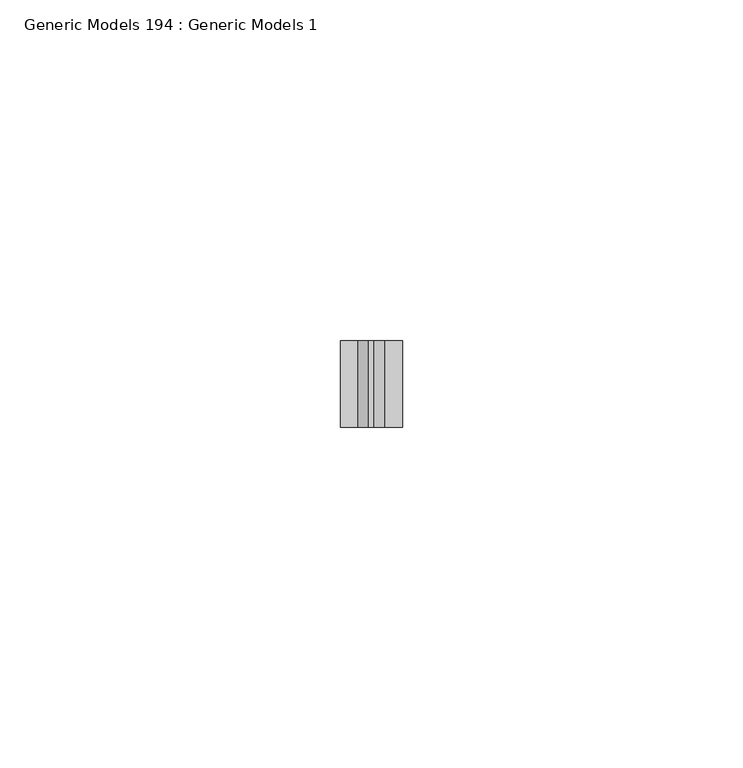
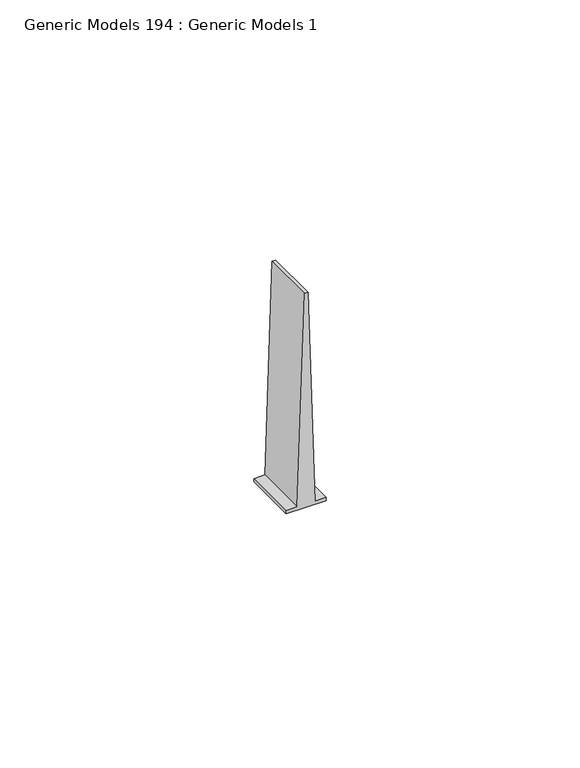
"""IFC4 building model written with IfcOpenShell, lengths in millimetres: proxy geometry, Generic Models 194 : Generic Models 1."""

import ifcopenshell
import ifcopenshell.guid

model = None  # the IFC model being written
_history = None  # IfcOwnerHistory: only IFC2X3 demands one
_inside = {}  # id of a spatial element -> (the spatial element, [elements in it])
_under = {}  # id of a project, library or spatial element -> (it, [spatial elements below it])
_declared = {}  # id of a project -> (the project, [libraries it declares])
_typed = {}  # id of a type object -> (the type object, [elements of that type])
_made_of = {}  # id of a material, layer set ... -> (it, [elements and type objects made of it])


def new_model(schema):
    """Start an empty IFC model of exactly this schema.

    Asked for "IFC4X3", IfcOpenShell would pick the latest addendum, in which some entities
    have other attributes; the version numbers below select the first issue.
    IFC2X3 requires an IfcOwnerHistory on every rooted entity: one is made here for all.
    """
    global model, _history
    if schema == "IFC4X3":
        model = ifcopenshell.file(schema_version=(4, 3, 0, 0))
    else:
        model = ifcopenshell.file(schema=schema)
    _inside.clear()
    _under.clear()
    _declared.clear()
    _typed.clear()
    _made_of.clear()
    _history = None
    if model.schema == "IFC2X3":
        org = make("IfcOrganization", Name="unknown")
        user = make(
            "IfcPersonAndOrganization",
            ThePerson=make("IfcPerson", FamilyName="unknown"),
            TheOrganization=org,
        )
        app = make(
            "IfcApplication",
            ApplicationDeveloper=org,
            Version="unknown",
            ApplicationFullName="unknown",
            ApplicationIdentifier="unknown",
        )
        _history = make(
            "IfcOwnerHistory",
            OwningUser=user,
            OwningApplication=app,
            ChangeAction="ADDED",
            CreationDate=0,
        )
    return model


def make(cls, **values):
    """One entity of the class cls with the attributes given. An attribute that is None is left unset."""
    return model.create_entity(
        cls, **{name: value for name, value in values.items() if value is not None}
    )


def rooted(cls, **values):
    """An entity with a GlobalId (a new one), such as an element, a storey or a relation."""
    return make(cls, GlobalId=ifcopenshell.guid.new(), OwnerHistory=_history, **values)


def si_unit(unit_type, name, prefix=None):
    """IfcSIUnit, for example si_unit("LENGTHUNIT", "METRE", prefix="MILLI")."""
    return make("IfcSIUnit", UnitType=unit_type, Prefix=prefix, Name=name)


def assignment(units):
    """IfcUnitAssignment: the units of a project."""
    return None if units is None else make("IfcUnitAssignment", Units=units)


def point(xyz):
    """IfcCartesianPoint."""
    return None if xyz is None else make("IfcCartesianPoint", Coordinates=xyz)


def direction(xyz):
    """IfcDirection."""
    return None if xyz is None else make("IfcDirection", DirectionRatios=xyz)


def frame(location, z_axis=None, x_axis=None):
    """IfcAxis2Placement3D, a coordinate frame: its origin and axes. An axis left out is left unset."""
    return make(
        "IfcAxis2Placement3D",
        Location=point(location),
        Axis=direction(z_axis),
        RefDirection=direction(x_axis),
    )


def origin():
    """The frame at (0, 0, 0) with its axes left unset."""
    return frame((0.0, 0.0, 0.0))


def place(relative_to, where):
    """IfcLocalPlacement: puts the frame where relative to a parent placement (None: the world)."""
    return make(
        "IfcLocalPlacement", PlacementRelTo=relative_to, RelativePlacement=where
    )


def context(
    kind, dimensions, precision=None, world=None, true_north=None, identifier=None
):
    """IfcGeometricRepresentationContext, for example the 3D "Model" context."""
    return make(
        "IfcGeometricRepresentationContext",
        ContextIdentifier=identifier,
        ContextType=kind,
        CoordinateSpaceDimension=dimensions,
        Precision=precision,
        WorldCoordinateSystem=world,
        TrueNorth=true_north,
    )


def project(units=None, contexts=None):
    """IfcProject with its units and contexts."""
    return rooted(
        "IfcProject",
        Name="project",
        RepresentationContexts=contexts,
        UnitsInContext=assignment(units),
    )


def spatial(cls, under=None, at=None, **own):
    """A site, building, storey or space (cls), placed at a placement, below another one or the project."""
    s = rooted(cls, ObjectPlacement=at, **own)
    if under is not None:
        _under.setdefault(under.id(), (under, []))[1].append(s)
    return s


def polyline(points):
    """IfcPolyline through the points."""
    return make("IfcPolyline", Points=[point(p) for p in points])


def outline(outer, holes=None, kind="AREA"):
    """IfcArbitraryClosedProfileDef: a profile drawn as a closed curve; with holes, ...WithVoids."""
    if holes is None:
        return make("IfcArbitraryClosedProfileDef", ProfileType=kind, OuterCurve=outer)
    return make(
        "IfcArbitraryProfileDefWithVoids",
        ProfileType=kind,
        OuterCurve=outer,
        InnerCurves=holes,
    )


def extrude(swept, where, along, depth):
    """IfcExtrudedAreaSolid: the profile swept, set in the frame where, extruded along a direction by depth."""
    return make(
        "IfcExtrudedAreaSolid",
        SweptArea=swept,
        Position=where,
        ExtrudedDirection=direction(along),
        Depth=depth,
    )


def shape(context_of_items, identifier, shape_type, items):
    """IfcShapeRepresentation: the items that make up one representation, for example the "Body"."""
    return make(
        "IfcShapeRepresentation",
        ContextOfItems=context_of_items,
        RepresentationIdentifier=identifier,
        RepresentationType=shape_type,
        Items=items,
    )


def source(mapping_origin, context_of_items, identifier, shape_type, items):
    """IfcRepresentationMap: a shape defined once, which mapped items show again and again."""
    return make(
        "IfcRepresentationMap",
        MappingOrigin=mapping_origin,
        MappedRepresentation=shape(context_of_items, identifier, shape_type, items),
    )


def transform(
    local_origin,
    x_axis=None,
    y_axis=None,
    z_axis=None,
    scale=None,
    scale2=None,
    scale3=None,
    uniform=True,
):
    """IfcCartesianTransformationOperator3D, or its non-uniform kind. x_axis, y_axis, z_axis: its Axis1, 2, 3."""
    if uniform:
        return make(
            "IfcCartesianTransformationOperator3D",
            Axis1=direction(x_axis),
            Axis2=direction(y_axis),
            LocalOrigin=point(local_origin),
            Scale=scale,
            Axis3=direction(z_axis),
        )
    return make(
        "IfcCartesianTransformationOperator3DnonUniform",
        Axis1=direction(x_axis),
        Axis2=direction(y_axis),
        LocalOrigin=point(local_origin),
        Scale=scale,
        Axis3=direction(z_axis),
        Scale2=scale2,
        Scale3=scale3,
    )


def mapped(mapping_source, mapping_target):
    """IfcMappedItem: shows the shape of a source again, moved by a transform."""
    return make(
        "IfcMappedItem", MappingSource=mapping_source, MappingTarget=mapping_target
    )


def made_of(thing, what):
    """Note that an element or type object is made of a material, layer set ...; save() writes the relation."""
    if what is not None:
        _made_of.setdefault(what.id(), (what, []))[1].append(thing)
    return thing


def element(
    cls,
    number,
    at=None,
    inside=None,
    cuts=None,
    type_object=None,
    material=None,
    context=None,
    identifier="Body",
    shape_type=None,
    held_by="IfcProductDefinitionShape",
    body=None,
    shapes=None,
    **own,
):
    """One element of the class cls, such as IfcWall. Its Tag is "e" and its number.

    at: its placement. inside: the storey or other place that contains it. cuts: it is an
    opening in that element (IfcRelVoidsElement). A single representation is given by context,
    identifier, shape_type and body (its items); several are given by shapes. held_by: the class
    of the entity that holds the representations. save() writes the other relations.
    """
    e = rooted(cls, Tag="e%d" % number, ObjectPlacement=at, **own)
    if body is not None:
        shapes = [shape(context, identifier, shape_type, body)]
    if shapes is not None:
        e.Representation = make(held_by, Representations=shapes)
    if inside is not None:
        _inside.setdefault(inside.id(), (inside, []))[1].append(e)
    if cuts is not None:
        rooted(
            "IfcRelVoidsElement", RelatingBuildingElement=cuts, RelatedOpeningElement=e
        )
    if type_object is not None:
        _typed.setdefault(type_object.id(), (type_object, []))[1].append(e)
    return made_of(e, material)


def aggregate(whole, parts):
    """IfcRelAggregates: a whole, such as a stair, and the parts it consists of."""
    return rooted("IfcRelAggregates", RelatingObject=whole, RelatedObjects=parts)


def save(model, path):
    """Write the relations noted so far, then the file.

    IfcRelAggregates (storeys below a building ...), IfcRelContainedInSpatialStructure (elements
    in a storey), IfcRelDefinesByType, IfcRelAssociatesMaterial and IfcRelDeclares: one each for
    every whole, place, type object, material and project.
    """
    for whole, parts in _under.values():
        aggregate(whole, parts)
    for where, things in _inside.values():
        rooted(
            "IfcRelContainedInSpatialStructure",
            RelatedElements=things,
            RelatingStructure=where,
        )
    for kind, things in _typed.values():
        rooted("IfcRelDefinesByType", RelatedObjects=things, RelatingType=kind)
    for what, things in _made_of.values():
        rooted("IfcRelAssociatesMaterial", RelatedObjects=things, RelatingMaterial=what)
    for by, libraries in _declared.values():
        rooted("IfcRelDeclares", RelatingContext=by, RelatedDefinitions=libraries)
    model.write(path)


def generic_models_194_generic_models_1_34d9de7f(model_context):
    return source(origin(), model_context, "Body", "SweptSolid", [
        extrude(outline(polyline([(2455.06875, 49733.4159), (2455.06875, 49742.5091), (2455.8625, 49742.5091), (2455.8625, 49739.9592364), (2506.6625, 49738.3618473), (2506.6625, 49737.5631527), (2455.8625, 49735.9657636), (2455.8625, 49733.4159), (2455.06875, 49733.4159)])), frame((0.0, 565.15, 0.0), z_axis=(0.0, 1.0, 0.0), x_axis=(0.0, 0.0, 1.0)), (0.0, 0.0, 1.0), 12.7),
    ])


if __name__ == "__main__":
    model = new_model("IFC4")
    model_context = context("Model", 3, world=origin())
    ifc_project = project(units=[si_unit("LENGTHUNIT", "METRE", prefix="MILLI")], contexts=[model_context])
    site = spatial("IfcSite", under=ifc_project)
    building = spatial("IfcBuilding", under=site)
    placement = place(None, origin())
    generic_models_194_generic_models_1_shape = generic_models_194_generic_models_1_34d9de7f(model_context)
    element("IfcBuildingElementProxy", 1, Name="Generic Models 194 : Generic Models 1", ObjectType="Generic Models 194 : Generic Models 1", at=placement, inside=building, context=model_context, shape_type="MappedRepresentation", body=[
        mapped(generic_models_194_generic_models_1_shape, transform((0.0, 0.0, 0.0), x_axis=(1.0, 0.0, 0.0), y_axis=(0.0, 1.0, 0.0), z_axis=(0.0, 0.0, 1.0))),
    ])
    save(model, "model.ifc")

# Revit data of these elements
# Element 1 (IfcBuildingElementProxy, "Generic Models 194 : Generic Models 1")
#   Materials on its faces: "METAL RUNNER CHANNEL; FASTEN @ 24\" O.C."
# Materials
#   "METAL RUNNER CHANNEL; FASTEN @ 24\" O.C.": class "Unassigned", colour RGB 210 209 208, transparency 0, Keynote = "M05121300.02", Cost = 0
